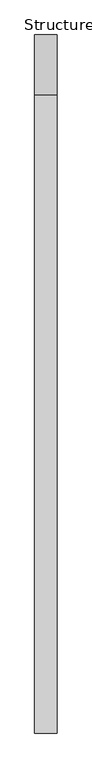
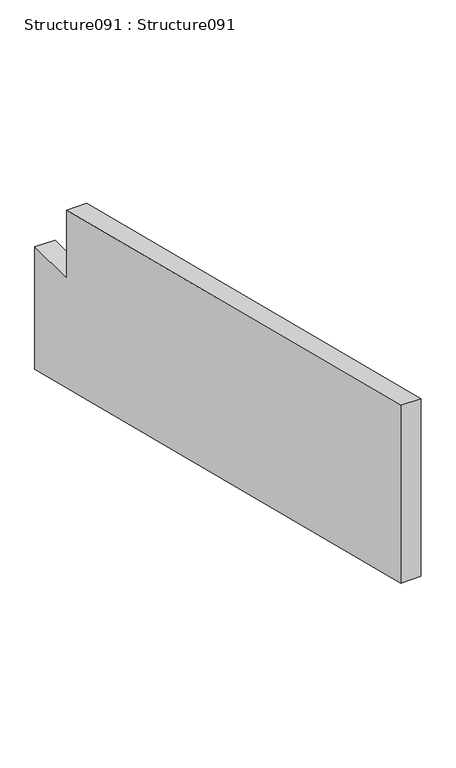
"""IFC4 building model written with IfcOpenShell, lengths in millimetres: proxy geometry, Structure091 : Structure091."""

import ifcopenshell
import ifcopenshell.guid

model = None  # the IFC model being written
_history = None  # IfcOwnerHistory: only IFC2X3 demands one
_inside = {}  # id of a spatial element -> (the spatial element, [elements in it])
_under = {}  # id of a project, library or spatial element -> (it, [spatial elements below it])
_declared = {}  # id of a project -> (the project, [libraries it declares])
_typed = {}  # id of a type object -> (the type object, [elements of that type])
_made_of = {}  # id of a material, layer set ... -> (it, [elements and type objects made of it])


def new_model(schema):
    """Start an empty IFC model of exactly this schema.

    Asked for "IFC4X3", IfcOpenShell would pick the latest addendum, in which some entities
    have other attributes; the version numbers below select the first issue.
    IFC2X3 requires an IfcOwnerHistory on every rooted entity: one is made here for all.
    """
    global model, _history
    if schema == "IFC4X3":
        model = ifcopenshell.file(schema_version=(4, 3, 0, 0))
    else:
        model = ifcopenshell.file(schema=schema)
    _inside.clear()
    _under.clear()
    _declared.clear()
    _typed.clear()
    _made_of.clear()
    _history = None
    if model.schema == "IFC2X3":
        org = make("IfcOrganization", Name="unknown")
        user = make(
            "IfcPersonAndOrganization",
            ThePerson=make("IfcPerson", FamilyName="unknown"),
            TheOrganization=org,
        )
        app = make(
            "IfcApplication",
            ApplicationDeveloper=org,
            Version="unknown",
            ApplicationFullName="unknown",
            ApplicationIdentifier="unknown",
        )
        _history = make(
            "IfcOwnerHistory",
            OwningUser=user,
            OwningApplication=app,
            ChangeAction="ADDED",
            CreationDate=0,
        )
    return model


def make(cls, **values):
    """One entity of the class cls with the attributes given. An attribute that is None is left unset."""
    return model.create_entity(
        cls, **{name: value for name, value in values.items() if value is not None}
    )


def rooted(cls, **values):
    """An entity with a GlobalId (a new one), such as an element, a storey or a relation."""
    return make(cls, GlobalId=ifcopenshell.guid.new(), OwnerHistory=_history, **values)


def si_unit(unit_type, name, prefix=None):
    """IfcSIUnit, for example si_unit("LENGTHUNIT", "METRE", prefix="MILLI")."""
    return make("IfcSIUnit", UnitType=unit_type, Prefix=prefix, Name=name)


def assignment(units):
    """IfcUnitAssignment: the units of a project."""
    return None if units is None else make("IfcUnitAssignment", Units=units)


def point(xyz):
    """IfcCartesianPoint."""
    return None if xyz is None else make("IfcCartesianPoint", Coordinates=xyz)


def direction(xyz):
    """IfcDirection."""
    return None if xyz is None else make("IfcDirection", DirectionRatios=xyz)


def frame(location, z_axis=None, x_axis=None):
    """IfcAxis2Placement3D, a coordinate frame: its origin and axes. An axis left out is left unset."""
    return make(
        "IfcAxis2Placement3D",
        Location=point(location),
        Axis=direction(z_axis),
        RefDirection=direction(x_axis),
    )


def origin():
    """The frame at (0, 0, 0) with its axes left unset."""
    return frame((0.0, 0.0, 0.0))


def place(relative_to, where):
    """IfcLocalPlacement: puts the frame where relative to a parent placement (None: the world)."""
    return make(
        "IfcLocalPlacement", PlacementRelTo=relative_to, RelativePlacement=where
    )


def context(
    kind, dimensions, precision=None, world=None, true_north=None, identifier=None
):
    """IfcGeometricRepresentationContext, for example the 3D "Model" context."""
    return make(
        "IfcGeometricRepresentationContext",
        ContextIdentifier=identifier,
        ContextType=kind,
        CoordinateSpaceDimension=dimensions,
        Precision=precision,
        WorldCoordinateSystem=world,
        TrueNorth=true_north,
    )


def project(units=None, contexts=None):
    """IfcProject with its units and contexts."""
    return rooted(
        "IfcProject",
        Name="project",
        RepresentationContexts=contexts,
        UnitsInContext=assignment(units),
    )


def spatial(cls, under=None, at=None, **own):
    """A site, building, storey or space (cls), placed at a placement, below another one or the project."""
    s = rooted(cls, ObjectPlacement=at, **own)
    if under is not None:
        _under.setdefault(under.id(), (under, []))[1].append(s)
    return s


def polyline(points):
    """IfcPolyline through the points."""
    return make("IfcPolyline", Points=[point(p) for p in points])


def outline(outer, holes=None, kind="AREA"):
    """IfcArbitraryClosedProfileDef: a profile drawn as a closed curve; with holes, ...WithVoids."""
    if holes is None:
        return make("IfcArbitraryClosedProfileDef", ProfileType=kind, OuterCurve=outer)
    return make(
        "IfcArbitraryProfileDefWithVoids",
        ProfileType=kind,
        OuterCurve=outer,
        InnerCurves=holes,
    )


def extrude(swept, where, along, depth):
    """IfcExtrudedAreaSolid: the profile swept, set in the frame where, extruded along a direction by depth."""
    return make(
        "IfcExtrudedAreaSolid",
        SweptArea=swept,
        Position=where,
        ExtrudedDirection=direction(along),
        Depth=depth,
    )


def shape(context_of_items, identifier, shape_type, items):
    """IfcShapeRepresentation: the items that make up one representation, for example the "Body"."""
    return make(
        "IfcShapeRepresentation",
        ContextOfItems=context_of_items,
        RepresentationIdentifier=identifier,
        RepresentationType=shape_type,
        Items=items,
    )


def source(mapping_origin, context_of_items, identifier, shape_type, items):
    """IfcRepresentationMap: a shape defined once, which mapped items show again and again."""
    return make(
        "IfcRepresentationMap",
        MappingOrigin=mapping_origin,
        MappedRepresentation=shape(context_of_items, identifier, shape_type, items),
    )


def transform(
    local_origin,
    x_axis=None,
    y_axis=None,
    z_axis=None,
    scale=None,
    scale2=None,
    scale3=None,
    uniform=True,
):
    """IfcCartesianTransformationOperator3D, or its non-uniform kind. x_axis, y_axis, z_axis: its Axis1, 2, 3."""
    if uniform:
        return make(
            "IfcCartesianTransformationOperator3D",
            Axis1=direction(x_axis),
            Axis2=direction(y_axis),
            LocalOrigin=point(local_origin),
            Scale=scale,
            Axis3=direction(z_axis),
        )
    return make(
        "IfcCartesianTransformationOperator3DnonUniform",
        Axis1=direction(x_axis),
        Axis2=direction(y_axis),
        LocalOrigin=point(local_origin),
        Scale=scale,
        Axis3=direction(z_axis),
        Scale2=scale2,
        Scale3=scale3,
    )


def mapped(mapping_source, mapping_target):
    """IfcMappedItem: shows the shape of a source again, moved by a transform."""
    return make(
        "IfcMappedItem", MappingSource=mapping_source, MappingTarget=mapping_target
    )


def made_of(thing, what):
    """Note that an element or type object is made of a material, layer set ...; save() writes the relation."""
    if what is not None:
        _made_of.setdefault(what.id(), (what, []))[1].append(thing)
    return thing


def element(
    cls,
    number,
    at=None,
    inside=None,
    cuts=None,
    type_object=None,
    material=None,
    context=None,
    identifier="Body",
    shape_type=None,
    held_by="IfcProductDefinitionShape",
    body=None,
    shapes=None,
    **own,
):
    """One element of the class cls, such as IfcWall. Its Tag is "e" and its number.

    at: its placement. inside: the storey or other place that contains it. cuts: it is an
    opening in that element (IfcRelVoidsElement). A single representation is given by context,
    identifier, shape_type and body (its items); several are given by shapes. held_by: the class
    of the entity that holds the representations. save() writes the other relations.
    """
    e = rooted(cls, Tag="e%d" % number, ObjectPlacement=at, **own)
    if body is not None:
        shapes = [shape(context, identifier, shape_type, body)]
    if shapes is not None:
        e.Representation = make(held_by, Representations=shapes)
    if inside is not None:
        _inside.setdefault(inside.id(), (inside, []))[1].append(e)
    if cuts is not None:
        rooted(
            "IfcRelVoidsElement", RelatingBuildingElement=cuts, RelatedOpeningElement=e
        )
    if type_object is not None:
        _typed.setdefault(type_object.id(), (type_object, []))[1].append(e)
    return made_of(e, material)


def aggregate(whole, parts):
    """IfcRelAggregates: a whole, such as a stair, and the parts it consists of."""
    return rooted("IfcRelAggregates", RelatingObject=whole, RelatedObjects=parts)


def save(model, path):
    """Write the relations noted so far, then the file.

    IfcRelAggregates (storeys below a building ...), IfcRelContainedInSpatialStructure (elements
    in a storey), IfcRelDefinesByType, IfcRelAssociatesMaterial and IfcRelDeclares: one each for
    every whole, place, type object, material and project.
    """
    for whole, parts in _under.values():
        aggregate(whole, parts)
    for where, things in _inside.values():
        rooted(
            "IfcRelContainedInSpatialStructure",
            RelatedElements=things,
            RelatingStructure=where,
        )
    for kind, things in _typed.values():
        rooted("IfcRelDefinesByType", RelatedObjects=things, RelatingType=kind)
    for what, things in _made_of.values():
        rooted("IfcRelAssociatesMaterial", RelatedObjects=things, RelatingMaterial=what)
    for by, libraries in _declared.values():
        rooted("IfcRelDeclares", RelatingContext=by, RelatedDefinitions=libraries)
    model.write(path)


def structure091_structure091_83a2f42a(model_context):
    return source(origin(), model_context, "Body", "SweptSolid", [
        extrude(outline(polyline([(3064.0857256, 41796.3564587), (4341.2743993, 41477.0623881), (4341.2743993, 41318.4021881), (4461.9244012, 41318.4021881), (4461.9244012, 41032.8236949), (3064.0857256, 41382.2833638), (3064.0857256, 41796.3564587)])), frame((1414.2864664, 0.0, 0.0), z_axis=(1.0, 0.0, 0.0), x_axis=(0.0, 1.0, 0.0)), (0.0, 0.0, 1.0), 44.45),
    ])


if __name__ == "__main__":
    model = new_model("IFC4")
    model_context = context("Model", 3, world=origin())
    ifc_project = project(units=[si_unit("LENGTHUNIT", "METRE", prefix="MILLI")], contexts=[model_context])
    site = spatial("IfcSite", under=ifc_project)
    building = spatial("IfcBuilding", under=site)
    placement = place(None, origin())
    structure091_structure091_shape = structure091_structure091_83a2f42a(model_context)
    element("IfcBuildingElementProxy", 1, Name="Structure091 : Structure091", ObjectType="Structure091 : Structure091", at=placement, inside=building, context=model_context, shape_type="MappedRepresentation", body=[
        mapped(structure091_structure091_shape, transform((0.0, 0.0, 0.0), x_axis=(1.0, 0.0, 0.0), y_axis=(0.0, 1.0, 0.0), z_axis=(0.0, 0.0, 1.0))),
    ])
    save(model, "model.ifc")

# Revit data of these elements
# Type "Structure091 : Structure091"
#   NameOverride = "Structure091"
# Element 1 (IfcBuildingElementProxy, "Structure091 : Structure091")
#   Materials on its faces: "STRUCTURAL MEMBER (SEE DWGS)"
# Materials
#   "STRUCTURAL MEMBER (SEE DWGS)": class "Unassigned", colour RGB 214 178 158, transparency 0, Cost = 0
